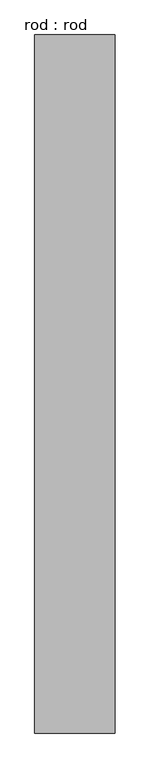
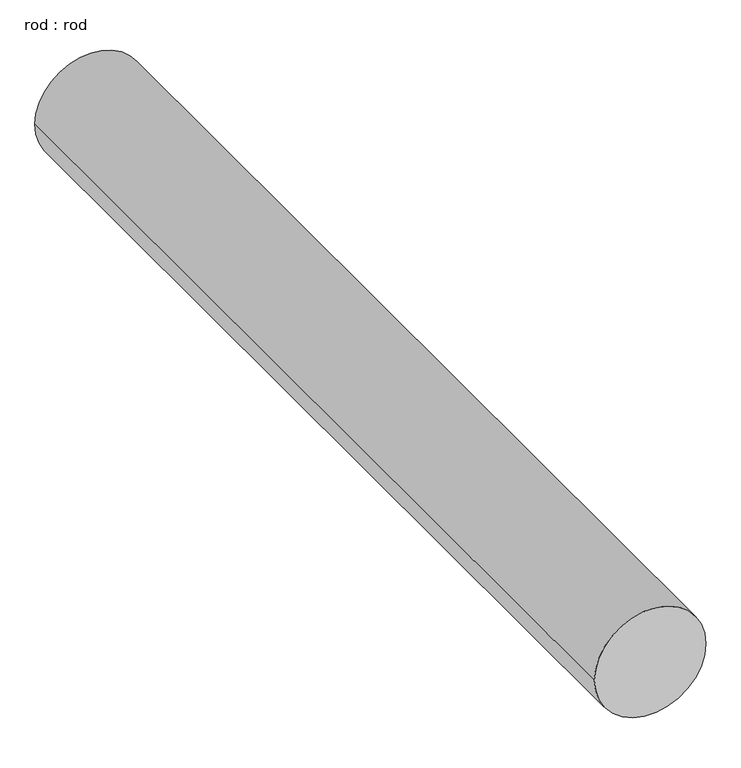
"""IFC4 building model written with IfcOpenShell, lengths in millimetres: proxy geometry, rod : rod."""

from ifc_helpers import new_model, si_unit, point, frame, frame_2d, origin, place, context, project, spatial, circle_curve, trimmed, segment, composite_curve, outline, extrude, source, transform, mapped, element, save


def rod_rod_2acd93f8(model_context):
    return source(origin(), model_context, "Body", "SweptSolid", [
        extrude(outline(composite_curve([segment(trimmed(circle_curve(frame_2d((0.0108462, 0.0)), 200.0), [point((0.0108462, 200.0))], [point((0.0108462, -200.0))], False, "CARTESIAN"), True, "CONTINUOUS"), segment(trimmed(circle_curve(frame_2d((0.0108462, 0.0)), 200.0), [point((0.0108462, -200.0))], [point((0.0108462, 200.0))], False, "CARTESIAN"), True, "CONTINUOUS")], self_intersect=False)), frame((0.0, 2352.7286153, 0.0), z_axis=(0.0, 1.0, 0.0), x_axis=(0.0, 0.0, 1.0)), (0.0, 0.0, 1.0), 3480.0),
    ])


if __name__ == "__main__":
    model = new_model("IFC4")
    model_context = context("Model", 3, world=origin())
    ifc_project = project(units=[si_unit("LENGTHUNIT", "METRE", prefix="MILLI")], contexts=[model_context])
    site = spatial("IfcSite", under=ifc_project)
    building = spatial("IfcBuilding", under=site)
    placement = place(None, origin())
    rod_rod_shape = rod_rod_2acd93f8(model_context)
    element("IfcBuildingElementProxy", 1, Name="rod : rod", ObjectType="rod : rod", at=placement, inside=building, context=model_context, shape_type="MappedRepresentation", body=[
        mapped(rod_rod_shape, transform((0.0, 0.0, 0.0), x_axis=(1.0, 0.0, 0.0), y_axis=(0.0, 1.0, 0.0), z_axis=(0.0, 0.0, 1.0))),
    ])
    save(model, "model.ifc")

# Revit data of these elements
# Type "rod : rod"
#   Default Elevation = 0
